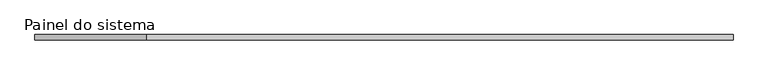
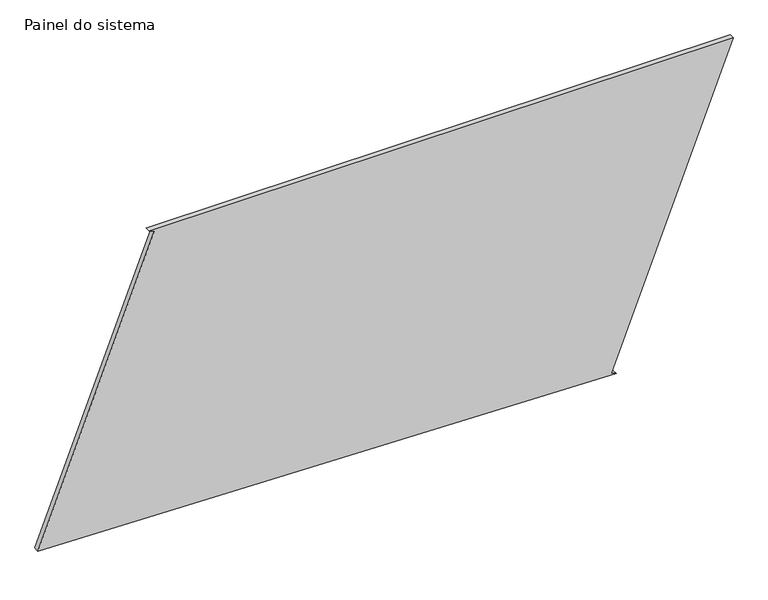
"""IFC4 building model written with IfcOpenShell, lengths in millimetres: plate geometry, Painel do sistema : Envidraçado."""

import ifcopenshell
import ifcopenshell.guid

model = None  # the IFC model being written
_history = None  # IfcOwnerHistory: only IFC2X3 demands one
_inside = {}  # id of a spatial element -> (the spatial element, [elements in it])
_under = {}  # id of a project, library or spatial element -> (it, [spatial elements below it])
_declared = {}  # id of a project -> (the project, [libraries it declares])
_typed = {}  # id of a type object -> (the type object, [elements of that type])
_made_of = {}  # id of a material, layer set ... -> (it, [elements and type objects made of it])


def new_model(schema):
    """Start an empty IFC model of exactly this schema.

    Asked for "IFC4X3", IfcOpenShell would pick the latest addendum, in which some entities
    have other attributes; the version numbers below select the first issue.
    IFC2X3 requires an IfcOwnerHistory on every rooted entity: one is made here for all.
    """
    global model, _history
    if schema == "IFC4X3":
        model = ifcopenshell.file(schema_version=(4, 3, 0, 0))
    else:
        model = ifcopenshell.file(schema=schema)
    _inside.clear()
    _under.clear()
    _declared.clear()
    _typed.clear()
    _made_of.clear()
    _history = None
    if model.schema == "IFC2X3":
        org = make("IfcOrganization", Name="unknown")
        user = make(
            "IfcPersonAndOrganization",
            ThePerson=make("IfcPerson", FamilyName="unknown"),
            TheOrganization=org,
        )
        app = make(
            "IfcApplication",
            ApplicationDeveloper=org,
            Version="unknown",
            ApplicationFullName="unknown",
            ApplicationIdentifier="unknown",
        )
        _history = make(
            "IfcOwnerHistory",
            OwningUser=user,
            OwningApplication=app,
            ChangeAction="ADDED",
            CreationDate=0,
        )
    return model


def make(cls, **values):
    """One entity of the class cls with the attributes given. An attribute that is None is left unset."""
    return model.create_entity(
        cls, **{name: value for name, value in values.items() if value is not None}
    )


def rooted(cls, **values):
    """An entity with a GlobalId (a new one), such as an element, a storey or a relation."""
    return make(cls, GlobalId=ifcopenshell.guid.new(), OwnerHistory=_history, **values)


def si_unit(unit_type, name, prefix=None):
    """IfcSIUnit, for example si_unit("LENGTHUNIT", "METRE", prefix="MILLI")."""
    return make("IfcSIUnit", UnitType=unit_type, Prefix=prefix, Name=name)


def assignment(units):
    """IfcUnitAssignment: the units of a project."""
    return None if units is None else make("IfcUnitAssignment", Units=units)


def point(xyz):
    """IfcCartesianPoint."""
    return None if xyz is None else make("IfcCartesianPoint", Coordinates=xyz)


def direction(xyz):
    """IfcDirection."""
    return None if xyz is None else make("IfcDirection", DirectionRatios=xyz)


def frame(location, z_axis=None, x_axis=None):
    """IfcAxis2Placement3D, a coordinate frame: its origin and axes. An axis left out is left unset."""
    return make(
        "IfcAxis2Placement3D",
        Location=point(location),
        Axis=direction(z_axis),
        RefDirection=direction(x_axis),
    )


def origin():
    """The frame at (0, 0, 0) with its axes left unset."""
    return frame((0.0, 0.0, 0.0))


def place(relative_to, where):
    """IfcLocalPlacement: puts the frame where relative to a parent placement (None: the world)."""
    return make(
        "IfcLocalPlacement", PlacementRelTo=relative_to, RelativePlacement=where
    )


def context(
    kind, dimensions, precision=None, world=None, true_north=None, identifier=None
):
    """IfcGeometricRepresentationContext, for example the 3D "Model" context."""
    return make(
        "IfcGeometricRepresentationContext",
        ContextIdentifier=identifier,
        ContextType=kind,
        CoordinateSpaceDimension=dimensions,
        Precision=precision,
        WorldCoordinateSystem=world,
        TrueNorth=true_north,
    )


def project(units=None, contexts=None):
    """IfcProject with its units and contexts."""
    return rooted(
        "IfcProject",
        Name="project",
        RepresentationContexts=contexts,
        UnitsInContext=assignment(units),
    )


def spatial(cls, under=None, at=None, **own):
    """A site, building, storey or space (cls), placed at a placement, below another one or the project."""
    s = rooted(cls, ObjectPlacement=at, **own)
    if under is not None:
        _under.setdefault(under.id(), (under, []))[1].append(s)
    return s


def polyline(points):
    """IfcPolyline through the points."""
    return make("IfcPolyline", Points=[point(p) for p in points])


def outline(outer, holes=None, kind="AREA"):
    """IfcArbitraryClosedProfileDef: a profile drawn as a closed curve; with holes, ...WithVoids."""
    if holes is None:
        return make("IfcArbitraryClosedProfileDef", ProfileType=kind, OuterCurve=outer)
    return make(
        "IfcArbitraryProfileDefWithVoids",
        ProfileType=kind,
        OuterCurve=outer,
        InnerCurves=holes,
    )


def extrude(swept, where, along, depth):
    """IfcExtrudedAreaSolid: the profile swept, set in the frame where, extruded along a direction by depth."""
    return make(
        "IfcExtrudedAreaSolid",
        SweptArea=swept,
        Position=where,
        ExtrudedDirection=direction(along),
        Depth=depth,
    )


def shape(context_of_items, identifier, shape_type, items):
    """IfcShapeRepresentation: the items that make up one representation, for example the "Body"."""
    return make(
        "IfcShapeRepresentation",
        ContextOfItems=context_of_items,
        RepresentationIdentifier=identifier,
        RepresentationType=shape_type,
        Items=items,
    )


def source(mapping_origin, context_of_items, identifier, shape_type, items):
    """IfcRepresentationMap: a shape defined once, which mapped items show again and again."""
    return make(
        "IfcRepresentationMap",
        MappingOrigin=mapping_origin,
        MappedRepresentation=shape(context_of_items, identifier, shape_type, items),
    )


def transform(
    local_origin,
    x_axis=None,
    y_axis=None,
    z_axis=None,
    scale=None,
    scale2=None,
    scale3=None,
    uniform=True,
):
    """IfcCartesianTransformationOperator3D, or its non-uniform kind. x_axis, y_axis, z_axis: its Axis1, 2, 3."""
    if uniform:
        return make(
            "IfcCartesianTransformationOperator3D",
            Axis1=direction(x_axis),
            Axis2=direction(y_axis),
            LocalOrigin=point(local_origin),
            Scale=scale,
            Axis3=direction(z_axis),
        )
    return make(
        "IfcCartesianTransformationOperator3DnonUniform",
        Axis1=direction(x_axis),
        Axis2=direction(y_axis),
        LocalOrigin=point(local_origin),
        Scale=scale,
        Axis3=direction(z_axis),
        Scale2=scale2,
        Scale3=scale3,
    )


def mapped(mapping_source, mapping_target):
    """IfcMappedItem: shows the shape of a source again, moved by a transform."""
    return make(
        "IfcMappedItem", MappingSource=mapping_source, MappingTarget=mapping_target
    )


def made_of(thing, what):
    """Note that an element or type object is made of a material, layer set ...; save() writes the relation."""
    if what is not None:
        _made_of.setdefault(what.id(), (what, []))[1].append(thing)
    return thing


def element(
    cls,
    number,
    at=None,
    inside=None,
    cuts=None,
    type_object=None,
    material=None,
    context=None,
    identifier="Body",
    shape_type=None,
    held_by="IfcProductDefinitionShape",
    body=None,
    shapes=None,
    **own,
):
    """One element of the class cls, such as IfcWall. Its Tag is "e" and its number.

    at: its placement. inside: the storey or other place that contains it. cuts: it is an
    opening in that element (IfcRelVoidsElement). A single representation is given by context,
    identifier, shape_type and body (its items); several are given by shapes. held_by: the class
    of the entity that holds the representations. save() writes the other relations.
    """
    e = rooted(cls, Tag="e%d" % number, ObjectPlacement=at, **own)
    if body is not None:
        shapes = [shape(context, identifier, shape_type, body)]
    if shapes is not None:
        e.Representation = make(held_by, Representations=shapes)
    if inside is not None:
        _inside.setdefault(inside.id(), (inside, []))[1].append(e)
    if cuts is not None:
        rooted(
            "IfcRelVoidsElement", RelatingBuildingElement=cuts, RelatedOpeningElement=e
        )
    if type_object is not None:
        _typed.setdefault(type_object.id(), (type_object, []))[1].append(e)
    return made_of(e, material)


def aggregate(whole, parts):
    """IfcRelAggregates: a whole, such as a stair, and the parts it consists of."""
    return rooted("IfcRelAggregates", RelatingObject=whole, RelatedObjects=parts)


def save(model, path):
    """Write the relations noted so far, then the file.

    IfcRelAggregates (storeys below a building ...), IfcRelContainedInSpatialStructure (elements
    in a storey), IfcRelDefinesByType, IfcRelAssociatesMaterial and IfcRelDeclares: one each for
    every whole, place, type object, material and project.
    """
    for whole, parts in _under.values():
        aggregate(whole, parts)
    for where, things in _inside.values():
        rooted(
            "IfcRelContainedInSpatialStructure",
            RelatedElements=things,
            RelatingStructure=where,
        )
    for kind, things in _typed.values():
        rooted("IfcRelDefinesByType", RelatedObjects=things, RelatingType=kind)
    for what, things in _made_of.values():
        rooted("IfcRelAssociatesMaterial", RelatedObjects=things, RelatingMaterial=what)
    for by, libraries in _declared.values():
        rooted("IfcRelDeclares", RelatingContext=by, RelatedDefinitions=libraries)
    model.write(path)


def painel_do_sistema_45333afa(model_context):
    return source(origin(), model_context, "Body", "SweptSolid", [
        extrude(outline(polyline([(0.0, 1080.0106281), (9.0972802, 1056.7245917), (1472.2661319, 1628.3485835), (1472.2661319, -1106.7980214), (1463.1688517, -1083.511985), (68.5668902, -1628.3485835), (0.0, 1080.0106281)])), frame((0.0, 24.5, 0.0), z_axis=(0.0, 1.0, 0.0), x_axis=(0.0, 0.0, 1.0)), (0.0, 0.0, 1.0), 25.0),
    ])


if __name__ == "__main__":
    model = new_model("IFC4")
    model_context = context("Model", 3, world=origin())
    ifc_project = project(units=[si_unit("LENGTHUNIT", "METRE", prefix="MILLI")], contexts=[model_context])
    site = spatial("IfcSite", under=ifc_project)
    building = spatial("IfcBuilding", under=site)
    placement = place(None, origin())
    painel_do_sistema_shape = painel_do_sistema_45333afa(model_context)
    element("IfcPlate", 1, ObjectType="Painel do sistema : Envidraçado", at=placement, inside=building, context=model_context, shape_type="MappedRepresentation", body=[
        mapped(painel_do_sistema_shape, transform((0.0, 0.0, 0.0), x_axis=(1.0, 0.0, 0.0), y_axis=(0.0, 1.0, 0.0), z_axis=(0.0, 0.0, 1.0))),
    ])
    save(model, "model.ifc")

# Revit data of these elements
# Type "Painel do sistema : Envidraçado"
#   Construction Type Id = "GSP4R"
#   Analytic Construction = "Vidraça única Pilkington 1/8 pol"
#   Visual Light Transmittance = 0.9
#   Solar Heat Gain Coefficient = 0.86
#   Heat Transfer Coefficient (U) = 6.7069 W/(m²·K)
# Element 1 (IfcPlate, "Painel do sistema : Envidraçado")
#   Materials on its faces: "Vidro"
# Materials
#   "Vidro": class "Vidro", colour RGB 0 128 192, transparency 0.9, Description = "Vidro de sílica", Cost = 0
